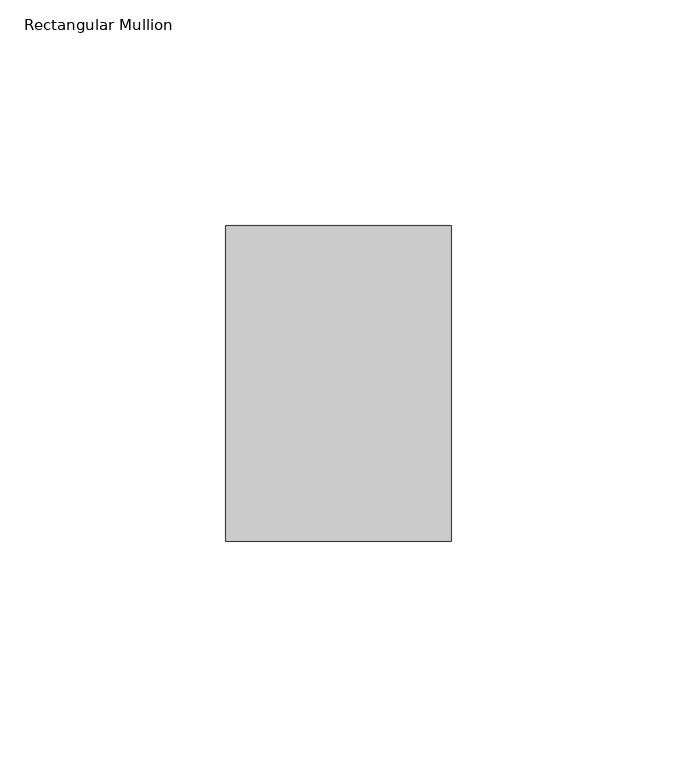
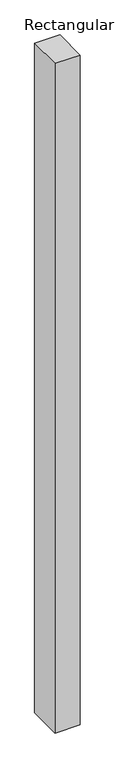
"""IFC4 building model written with IfcOpenShell, lengths in millimetres: member geometry, Rectangular Mullion : WWm-25x70-35mmOffset."""

from ifc_helpers import new_model, si_unit, frame, origin, place, context, project, spatial, polyline, outline, extrude, source, transform, mapped, element, save


def rectangular_mullion_e117e276(model_context):
    return source(origin(), model_context, "Body", "SweptSolid", [
        extrude(outline(polyline([(0.0, 0.0), (0.0, -70.0), (-50.0, -70.0), (-50.0, 0.0), (0.0, 0.0)])), frame((0.0, 0.0, -1410.3062061), z_axis=(0.0, 0.0, 1.0), x_axis=(1.0, 0.0, 0.0)), (0.0, 0.0, 1.0), 1410.3062061),
    ])


if __name__ == "__main__":
    model = new_model("IFC4")
    model_context = context("Model", 3, world=origin())
    ifc_project = project(units=[si_unit("LENGTHUNIT", "METRE", prefix="MILLI")], contexts=[model_context])
    site = spatial("IfcSite", under=ifc_project)
    building = spatial("IfcBuilding", under=site)
    placement = place(None, origin())
    rectangular_mullion_shape = rectangular_mullion_e117e276(model_context)
    element("IfcMember", 1, ObjectType="Rectangular Mullion : WWm-25x70-35mmOffset", at=placement, inside=building, context=model_context, shape_type="MappedRepresentation", body=[
        mapped(rectangular_mullion_shape, transform((0.0, 0.0, 0.0), x_axis=(1.0, 0.0, 0.0), y_axis=(0.0, 1.0, 0.0), z_axis=(0.0, 0.0, 1.0))),
    ])
    save(model, "model.ifc")

# Revit data of these elements
# Type "Rectangular Mullion : WWm-25x70-35mmOffset"
#   built-in parameter 1007351 = 0.114829 (stored number, unit not read)
#   built-in parameter 1007304 = 0.229659 (stored number, unit not read)
#   built-in parameter 1007301 = 0.082021 (stored number, unit not read)
#   built-in parameter 1007300 = 0.082021 (stored number, unit not read)
# Element 1 (IfcMember, "Rectangular Mullion : WWm-25x70-35mmOffset")
#   Materials on its faces: "WW-EC-RGB-Mullion"
# Materials
#   "WW-EC-RGB-Mullion": class "Generic", colour RGB 255 255 255, transparency 0, Comments = "If region requests black mullions, switch asset color to RGB 25-25-25", Description = "Generic Color", Cost = 0
